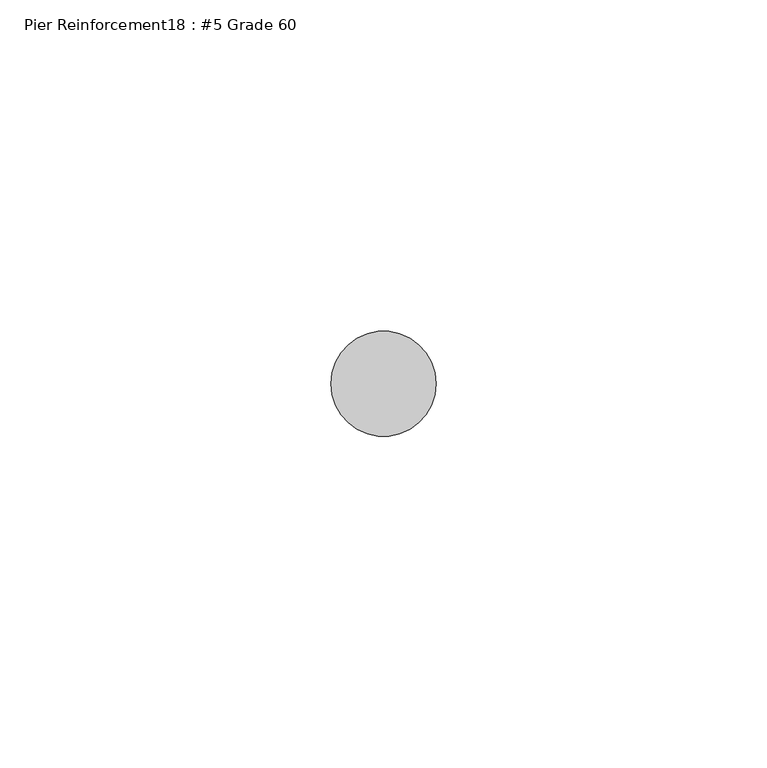
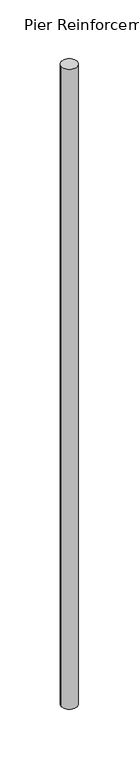
"""IFC4 building model written with IfcOpenShell, lengths in millimetres: proxy geometry, Pier Reinforcement18 : #5 Grade 60."""

from ifc_helpers import new_model, si_unit, point, frame, frame_2d, origin, place, context, project, spatial, circle_curve, trimmed, segment, composite_curve, outline, extrude, source, transform, mapped, element, save


def pier_reinforcement18_5_grade_60_3acffefc(model_context):
    return source(origin(), model_context, "Body", "SweptSolid", [
        extrude(outline(composite_curve([segment(trimmed(circle_curve(frame_2d((590226.0547365, -534096.6663841)), 7.9375), [point((590218.1172365, -534096.6663841))], [point((590233.9922365, -534096.6663841))], False, "CARTESIAN"), True, "CONTINUOUS"), segment(trimmed(circle_curve(frame_2d((590226.0547365, -534096.6663841)), 7.9375), [point((590233.9922365, -534096.6663841))], [point((590218.1172365, -534096.6663841))], False, "CARTESIAN"), True, "CONTINUOUS")], self_intersect=False)), frame((0.0, 0.0, -733.425), z_axis=(0.0, 0.0, 1.0), x_axis=(1.0, 0.0, 0.0)), (0.0, 0.0, 1.0), 685.8),
    ])


if __name__ == "__main__":
    model = new_model("IFC4")
    model_context = context("Model", 3, world=origin())
    ifc_project = project(units=[si_unit("LENGTHUNIT", "METRE", prefix="MILLI")], contexts=[model_context])
    site = spatial("IfcSite", under=ifc_project)
    building = spatial("IfcBuilding", under=site)
    placement = place(None, origin())
    pier_reinforcement18_5_grade_60_shape = pier_reinforcement18_5_grade_60_3acffefc(model_context)
    element("IfcBuildingElementProxy", 1, Name="Pier Reinforcement18 : #5 Grade 60", ObjectType="Pier Reinforcement18 : #5 Grade 60", at=placement, inside=building, context=model_context, shape_type="MappedRepresentation", body=[
        mapped(pier_reinforcement18_5_grade_60_shape, transform((0.0, 0.0, 0.0), x_axis=(1.0, 0.0, 0.0), y_axis=(0.0, 1.0, 0.0), z_axis=(0.0, 0.0, 1.0))),
    ])
    save(model, "model.ifc")

# Revit data of these elements
# Element 1 (IfcBuildingElementProxy, "Pier Reinforcement18 : #5 Grade 60")
#   Materials on its faces: "#4 GR. 60 REINF. @ 16\" O.C. EW."
# Materials
#   "#4 GR. 60 REINF. @ 16\" O.C. EW.": class "Generic", colour RGB 84 83 81, transparency 0, Cost = 0
